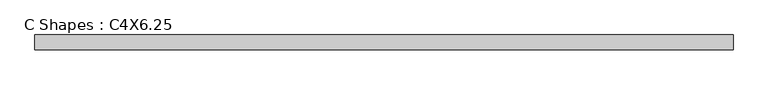
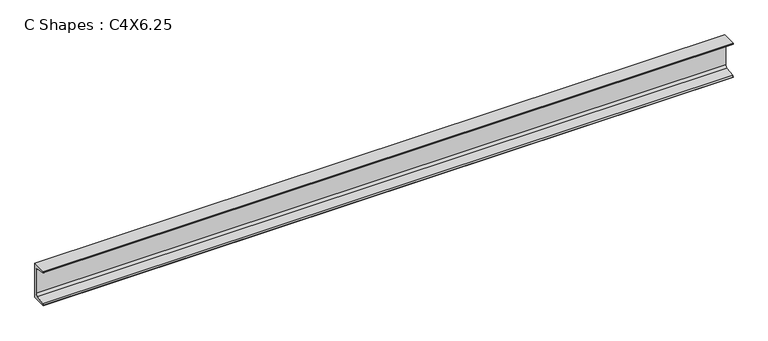
"""IFC4 building model written with IfcOpenShell, lengths in millimetres: beam geometry, C Shapes : C4X6.25."""

import ifcopenshell
import ifcopenshell.guid

model = None  # the IFC model being written
_history = None  # IfcOwnerHistory: only IFC2X3 demands one
_inside = {}  # id of a spatial element -> (the spatial element, [elements in it])
_under = {}  # id of a project, library or spatial element -> (it, [spatial elements below it])
_declared = {}  # id of a project -> (the project, [libraries it declares])
_typed = {}  # id of a type object -> (the type object, [elements of that type])
_made_of = {}  # id of a material, layer set ... -> (it, [elements and type objects made of it])


def new_model(schema):
    """Start an empty IFC model of exactly this schema.

    Asked for "IFC4X3", IfcOpenShell would pick the latest addendum, in which some entities
    have other attributes; the version numbers below select the first issue.
    IFC2X3 requires an IfcOwnerHistory on every rooted entity: one is made here for all.
    """
    global model, _history
    if schema == "IFC4X3":
        model = ifcopenshell.file(schema_version=(4, 3, 0, 0))
    else:
        model = ifcopenshell.file(schema=schema)
    _inside.clear()
    _under.clear()
    _declared.clear()
    _typed.clear()
    _made_of.clear()
    _history = None
    if model.schema == "IFC2X3":
        org = make("IfcOrganization", Name="unknown")
        user = make(
            "IfcPersonAndOrganization",
            ThePerson=make("IfcPerson", FamilyName="unknown"),
            TheOrganization=org,
        )
        app = make(
            "IfcApplication",
            ApplicationDeveloper=org,
            Version="unknown",
            ApplicationFullName="unknown",
            ApplicationIdentifier="unknown",
        )
        _history = make(
            "IfcOwnerHistory",
            OwningUser=user,
            OwningApplication=app,
            ChangeAction="ADDED",
            CreationDate=0,
        )
    return model


def make(cls, **values):
    """One entity of the class cls with the attributes given. An attribute that is None is left unset."""
    return model.create_entity(
        cls, **{name: value for name, value in values.items() if value is not None}
    )


def rooted(cls, **values):
    """An entity with a GlobalId (a new one), such as an element, a storey or a relation."""
    return make(cls, GlobalId=ifcopenshell.guid.new(), OwnerHistory=_history, **values)


def si_unit(unit_type, name, prefix=None):
    """IfcSIUnit, for example si_unit("LENGTHUNIT", "METRE", prefix="MILLI")."""
    return make("IfcSIUnit", UnitType=unit_type, Prefix=prefix, Name=name)


def assignment(units):
    """IfcUnitAssignment: the units of a project."""
    return None if units is None else make("IfcUnitAssignment", Units=units)


def point(xyz):
    """IfcCartesianPoint."""
    return None if xyz is None else make("IfcCartesianPoint", Coordinates=xyz)


def direction(xyz):
    """IfcDirection."""
    return None if xyz is None else make("IfcDirection", DirectionRatios=xyz)


def frame(location, z_axis=None, x_axis=None):
    """IfcAxis2Placement3D, a coordinate frame: its origin and axes. An axis left out is left unset."""
    return make(
        "IfcAxis2Placement3D",
        Location=point(location),
        Axis=direction(z_axis),
        RefDirection=direction(x_axis),
    )


def frame_2d(location, x_axis=None):
    """IfcAxis2Placement2D, a coordinate frame in the plane: its origin and x axis."""
    return make(
        "IfcAxis2Placement2D", Location=point(location), RefDirection=direction(x_axis)
    )


def origin():
    """The frame at (0, 0, 0) with its axes left unset."""
    return frame((0.0, 0.0, 0.0))


def place(relative_to, where):
    """IfcLocalPlacement: puts the frame where relative to a parent placement (None: the world)."""
    return make(
        "IfcLocalPlacement", PlacementRelTo=relative_to, RelativePlacement=where
    )


def context(
    kind, dimensions, precision=None, world=None, true_north=None, identifier=None
):
    """IfcGeometricRepresentationContext, for example the 3D "Model" context."""
    return make(
        "IfcGeometricRepresentationContext",
        ContextIdentifier=identifier,
        ContextType=kind,
        CoordinateSpaceDimension=dimensions,
        Precision=precision,
        WorldCoordinateSystem=world,
        TrueNorth=true_north,
    )


def project(units=None, contexts=None):
    """IfcProject with its units and contexts."""
    return rooted(
        "IfcProject",
        Name="project",
        RepresentationContexts=contexts,
        UnitsInContext=assignment(units),
    )


def spatial(cls, under=None, at=None, **own):
    """A site, building, storey or space (cls), placed at a placement, below another one or the project."""
    s = rooted(cls, ObjectPlacement=at, **own)
    if under is not None:
        _under.setdefault(under.id(), (under, []))[1].append(s)
    return s


def polyline(points):
    """IfcPolyline through the points."""
    return make("IfcPolyline", Points=[point(p) for p in points])


def circle_curve(where, radius):
    """IfcCircle in the frame where."""
    return make("IfcCircle", Position=where, Radius=radius)


def trimmed(basis, trim1, trim2, sense, master):
    """IfcTrimmedCurve: the piece of a basis curve between two trims."""
    return make(
        "IfcTrimmedCurve",
        BasisCurve=basis,
        Trim1=trim1,
        Trim2=trim2,
        SenseAgreement=sense,
        MasterRepresentation=master,
    )


def segment(curve, same_sense, transition):
    """IfcCompositeCurveSegment."""
    return make(
        "IfcCompositeCurveSegment",
        Transition=transition,
        SameSense=same_sense,
        ParentCurve=curve,
    )


def composite_curve(segments, self_intersect=None):
    """IfcCompositeCurve: segments joined end to end."""
    return make("IfcCompositeCurve", Segments=segments, SelfIntersect=self_intersect)


def outline(outer, holes=None, kind="AREA"):
    """IfcArbitraryClosedProfileDef: a profile drawn as a closed curve; with holes, ...WithVoids."""
    if holes is None:
        return make("IfcArbitraryClosedProfileDef", ProfileType=kind, OuterCurve=outer)
    return make(
        "IfcArbitraryProfileDefWithVoids",
        ProfileType=kind,
        OuterCurve=outer,
        InnerCurves=holes,
    )


def extrude(swept, where, along, depth):
    """IfcExtrudedAreaSolid: the profile swept, set in the frame where, extruded along a direction by depth."""
    return make(
        "IfcExtrudedAreaSolid",
        SweptArea=swept,
        Position=where,
        ExtrudedDirection=direction(along),
        Depth=depth,
    )


def shape(context_of_items, identifier, shape_type, items):
    """IfcShapeRepresentation: the items that make up one representation, for example the "Body"."""
    return make(
        "IfcShapeRepresentation",
        ContextOfItems=context_of_items,
        RepresentationIdentifier=identifier,
        RepresentationType=shape_type,
        Items=items,
    )


def source(mapping_origin, context_of_items, identifier, shape_type, items):
    """IfcRepresentationMap: a shape defined once, which mapped items show again and again."""
    return make(
        "IfcRepresentationMap",
        MappingOrigin=mapping_origin,
        MappedRepresentation=shape(context_of_items, identifier, shape_type, items),
    )


def transform(
    local_origin,
    x_axis=None,
    y_axis=None,
    z_axis=None,
    scale=None,
    scale2=None,
    scale3=None,
    uniform=True,
):
    """IfcCartesianTransformationOperator3D, or its non-uniform kind. x_axis, y_axis, z_axis: its Axis1, 2, 3."""
    if uniform:
        return make(
            "IfcCartesianTransformationOperator3D",
            Axis1=direction(x_axis),
            Axis2=direction(y_axis),
            LocalOrigin=point(local_origin),
            Scale=scale,
            Axis3=direction(z_axis),
        )
    return make(
        "IfcCartesianTransformationOperator3DnonUniform",
        Axis1=direction(x_axis),
        Axis2=direction(y_axis),
        LocalOrigin=point(local_origin),
        Scale=scale,
        Axis3=direction(z_axis),
        Scale2=scale2,
        Scale3=scale3,
    )


def mapped(mapping_source, mapping_target):
    """IfcMappedItem: shows the shape of a source again, moved by a transform."""
    return make(
        "IfcMappedItem", MappingSource=mapping_source, MappingTarget=mapping_target
    )


def made_of(thing, what):
    """Note that an element or type object is made of a material, layer set ...; save() writes the relation."""
    if what is not None:
        _made_of.setdefault(what.id(), (what, []))[1].append(thing)
    return thing


def element(
    cls,
    number,
    at=None,
    inside=None,
    cuts=None,
    type_object=None,
    material=None,
    context=None,
    identifier="Body",
    shape_type=None,
    held_by="IfcProductDefinitionShape",
    body=None,
    shapes=None,
    **own,
):
    """One element of the class cls, such as IfcWall. Its Tag is "e" and its number.

    at: its placement. inside: the storey or other place that contains it. cuts: it is an
    opening in that element (IfcRelVoidsElement). A single representation is given by context,
    identifier, shape_type and body (its items); several are given by shapes. held_by: the class
    of the entity that holds the representations. save() writes the other relations.
    """
    e = rooted(cls, Tag="e%d" % number, ObjectPlacement=at, **own)
    if body is not None:
        shapes = [shape(context, identifier, shape_type, body)]
    if shapes is not None:
        e.Representation = make(held_by, Representations=shapes)
    if inside is not None:
        _inside.setdefault(inside.id(), (inside, []))[1].append(e)
    if cuts is not None:
        rooted(
            "IfcRelVoidsElement", RelatingBuildingElement=cuts, RelatedOpeningElement=e
        )
    if type_object is not None:
        _typed.setdefault(type_object.id(), (type_object, []))[1].append(e)
    return made_of(e, material)


def aggregate(whole, parts):
    """IfcRelAggregates: a whole, such as a stair, and the parts it consists of."""
    return rooted("IfcRelAggregates", RelatingObject=whole, RelatedObjects=parts)


def save(model, path):
    """Write the relations noted so far, then the file.

    IfcRelAggregates (storeys below a building ...), IfcRelContainedInSpatialStructure (elements
    in a storey), IfcRelDefinesByType, IfcRelAssociatesMaterial and IfcRelDeclares: one each for
    every whole, place, type object, material and project.
    """
    for whole, parts in _under.values():
        aggregate(whole, parts)
    for where, things in _inside.values():
        rooted(
            "IfcRelContainedInSpatialStructure",
            RelatedElements=things,
            RelatingStructure=where,
        )
    for kind, things in _typed.values():
        rooted("IfcRelDefinesByType", RelatedObjects=things, RelatingType=kind)
    for what, things in _made_of.values():
        rooted("IfcRelAssociatesMaterial", RelatedObjects=things, RelatingMaterial=what)
    for by, libraries in _declared.values():
        rooted("IfcRelDeclares", RelatingContext=by, RelatedDefinitions=libraries)
    model.write(path)


def c_shapes_c4x6_25_a736a65e(model_context):
    return source(origin(), model_context, "Body", "SweptSolid", [
        extrude(outline(composite_curve([segment(polyline([(11.049, 50.8), (11.049, -50.8), (-30.861, -50.8), (-30.861, -49.7865772)]), True, "CONTINUOUS"), segment(trimmed(circle_curve(frame_2d((-27.4066, -49.7865772)), 3.4544), [point((-30.861, -49.7865772))], [point((-27.9743618, -46.379155))], False, "CARTESIAN"), True, "CONTINUOUS"), segment(polyline([(-27.9743618, -46.379155), (-0.9980765, -41.8842311)]), True, "CONTINUOUS"), segment(trimmed(circle_curve(frame_2d((-2.1336, -35.0693868)), 6.9088), [point((-0.9980765, -41.8842311))], [point((4.7752, -35.0693868))], True, "CARTESIAN"), True, "CONTINUOUS"), segment(polyline([(4.7752, -35.0693868), (4.7752, 35.0693868)]), True, "CONTINUOUS"), segment(trimmed(circle_curve(frame_2d((-2.1336, 35.0693868)), 6.9088), [point((4.7752, 35.0693868))], [point((-0.9980765, 41.8842311))], True, "CARTESIAN"), True, "CONTINUOUS"), segment(polyline([(-0.9980765, 41.8842311), (-27.9743618, 46.379155)]), True, "CONTINUOUS"), segment(trimmed(circle_curve(frame_2d((-27.4066, 49.7865772)), 3.4544), [point((-27.9743618, 46.379155))], [point((-30.861, 49.7865772))], False, "CARTESIAN"), True, "CONTINUOUS"), segment(polyline([(-30.861, 49.7865772), (-30.861, 50.8), (11.049, 50.8)]), True, "CONTINUOUS")], self_intersect=False)), frame((-974.344, 0.0, 0.0), z_axis=(1.0, 0.0, 0.0), x_axis=(0.0, 1.0, 0.0)), (0.0, 0.0, 1.0), 1948.688),
    ])


if __name__ == "__main__":
    model = new_model("IFC4")
    model_context = context("Model", 3, world=origin())
    ifc_project = project(units=[si_unit("LENGTHUNIT", "METRE", prefix="MILLI")], contexts=[model_context])
    site = spatial("IfcSite", under=ifc_project)
    building = spatial("IfcBuilding", under=site)
    placement = place(None, origin())
    c_shapes_c4x6_25_shape = c_shapes_c4x6_25_a736a65e(model_context)
    element("IfcBeam", 1, ObjectType="C Shapes : C4X6.25", at=placement, inside=building, context=model_context, shape_type="MappedRepresentation", body=[
        mapped(c_shapes_c4x6_25_shape, transform((0.0, 0.0, 0.0), x_axis=(1.0, 0.0, 0.0), y_axis=(0.0, 1.0, 0.0), z_axis=(0.0, 0.0, 1.0))),
    ])
    save(model, "model.ifc")

# Revit data of these elements
# Type "C Shapes : C4X6.25"
#   Section Name Key = "ChannelsC4X6.25"
#   Assembly Code = "B10"
#   Width = 1.650"
#   Web Thickness = 0.247"
#   Web Fillet = 0.272"
#   Warping Constant = 1.03 in⁶
#   Torsional Moment of Inertia = 0.0487 in⁴
#   Sloped Flange Angle = 9.46°
#   Section Area = 1.77 in²
#   Plastic Modulus weak axis = 0.569 in³
#   Plastic Modulus strong axis = 2.43 in³
#   Nominal Weight = 6.25 lbf/ft
#   Moment of Inertia weak axis = 0.345 in⁴
#   Moment of Inertia strong axis = 4.00 in⁴
#   Height = 4.000"
#   Flange Thickness Location = 0.7015"
#   Flange Thickness = 0.272"
#   Flange Fillet = 0.136"
#   Elastic Modulus weak axis = 0.284 in³
#   Elastic Modulus strong axis = 2.00 in³
#   Centroid Vertical = 2.000"
#   Centroid Horizontal = 0.435"
#   Length [instance default] = 5' - 0"
#   Structural Material [instance default] = Steel ASTM A36
#   Principal Axes Angle = 0
#   Bolt Spacing = 0
# Element 1 (IfcBeam, "C Shapes : C4X6.25")
#   Materials on its faces: "Steel ASTM A36"
# Materials
#   "Steel ASTM A36": class "Metal", colour RGB 199 199 199, transparency 0, Description = "Structural steel, ASTM A36 Grade B, mill finish", Cost = 0
